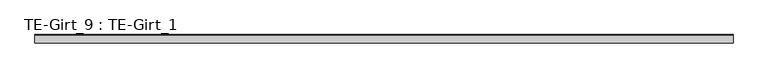
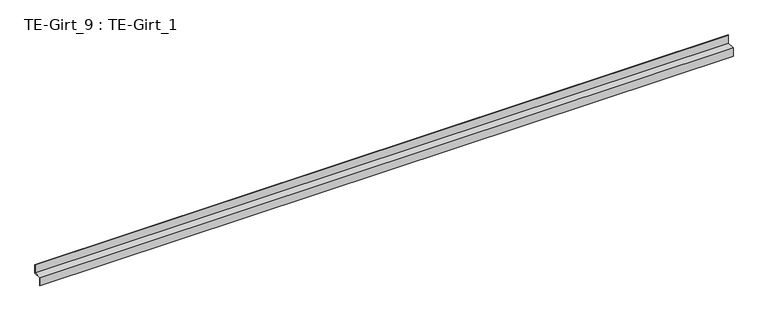
"""IFC4 building model written with IfcOpenShell, lengths in millimetres: proxy geometry, TE-Girt_9 : TE-Girt_1."""

from ifc_helpers import new_model, si_unit, frame, origin, place, context, project, spatial, polyline, outline, extrude, source, transform, mapped, element, save


def te_girt_9_te_girt_1_cbbea95c(model_context):
    return source(origin(), model_context, "Body", "SweptSolid", [
        extrude(outline(polyline([(-531639.2163841, 2374.9), (-531673.231966, 2374.9), (-531673.231966, 2337.6929688), (-531674.1249348, 2337.6929688), (-531674.1249348, 2375.7929688), (-531640.1093528, 2375.7929688), (-531640.1093528, 2413.0), (-531639.2163841, 2413.0), (-531639.2163841, 2374.9)])), frame((587365.3854739, 0.0, 0.0), z_axis=(1.0, 0.0, 0.0), x_axis=(0.0, 1.0, 0.0)), (0.0, 0.0, 1.0), 2953.258),
    ])


if __name__ == "__main__":
    model = new_model("IFC4")
    model_context = context("Model", 3, world=origin())
    ifc_project = project(units=[si_unit("LENGTHUNIT", "METRE", prefix="MILLI")], contexts=[model_context])
    site = spatial("IfcSite", under=ifc_project)
    building = spatial("IfcBuilding", under=site)
    placement = place(None, origin())
    te_girt_9_te_girt_1_shape = te_girt_9_te_girt_1_cbbea95c(model_context)
    element("IfcBuildingElementProxy", 1, Name="TE-Girt_9 : TE-Girt_1", ObjectType="TE-Girt_9 : TE-Girt_1", at=placement, inside=building, context=model_context, shape_type="MappedRepresentation", body=[
        mapped(te_girt_9_te_girt_1_shape, transform((0.0, 0.0, 0.0), x_axis=(1.0, 0.0, 0.0), y_axis=(0.0, 1.0, 0.0), z_axis=(0.0, 0.0, 1.0))),
    ])
    save(model, "model.ifc")

# Revit data of these elements
# Element 1 (IfcBuildingElementProxy, "TE-Girt_9 : TE-Girt_1")
#   Materials on its faces: "Z-FURRING, COLD-FORMED GALV."
# Materials
#   "Z-FURRING, COLD-FORMED GALV.": class "Generic", colour RGB 143 142 141, transparency 0, Cost = 0
